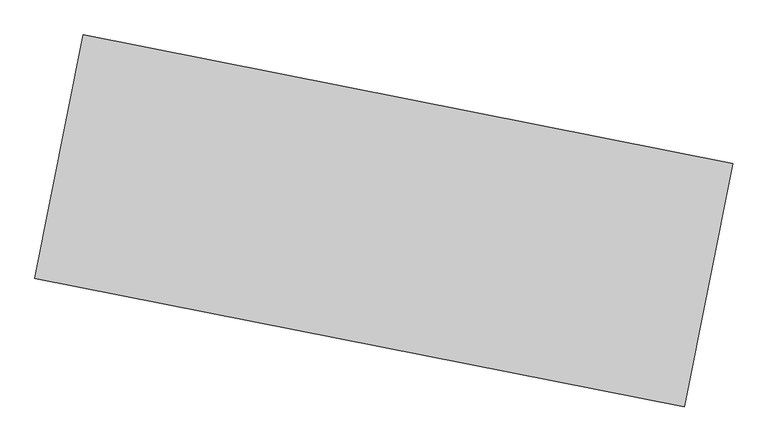
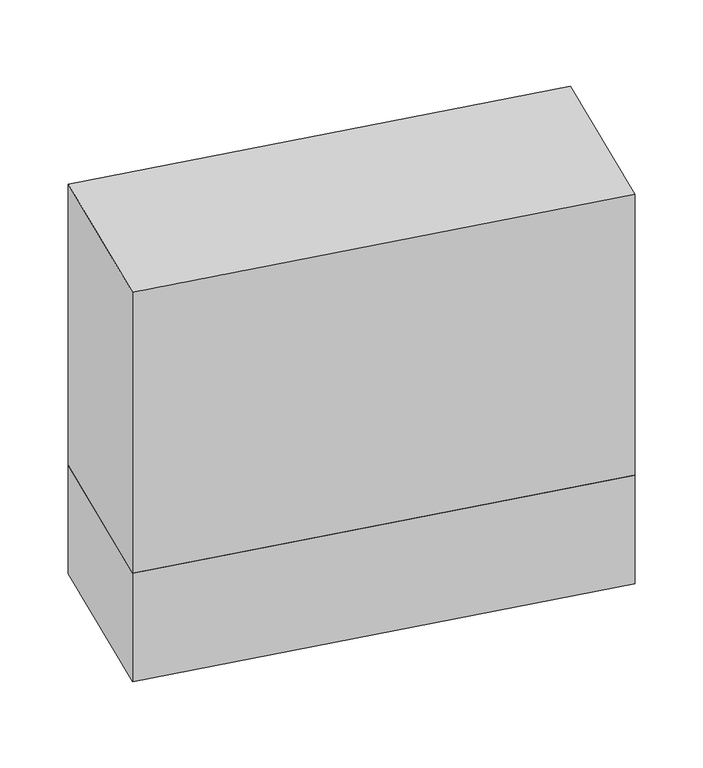
"""IFC4 building model written with IfcOpenShell, lengths in millimetres: furniture geometry, Monument sign2 : Monument sign."""

from ifc_helpers import new_model, si_unit, frame, origin, origin_with_axes, place, context, project, spatial, polyline, outline, extrude, source, transform, mapped, element, save


def furniture_524f5cd6(model_context):
    return source(origin(), model_context, "Body", "SweptSolid", [
        extrude(outline(polyline([(-3303.1352684, 235123.304702), (-911.1604416, 234649.7532396), (-1088.74224, 233752.7626795), (-3480.7170669, 234226.314142), (-3303.1352684, 235123.304702)])), origin_with_axes(), (0.0, 0.0, 1.0), 1574.8),
        extrude(outline(polyline([(-911.1604416, 234649.7532396), (-1088.74224, 233752.7626795), (-3480.7170669, 234226.314142), (-3303.1352684, 235123.304702), (-911.1604416, 234649.7532396)])), frame((0.0, 0.0, -609.6), z_axis=(0.0, 0.0, 1.0), x_axis=(1.0, 0.0, 0.0)), (0.0, 0.0, 1.0), 609.6),
    ])


if __name__ == "__main__":
    model = new_model("IFC4")
    model_context = context("Model", 3, world=origin())
    ifc_project = project(units=[si_unit("LENGTHUNIT", "METRE", prefix="MILLI")], contexts=[model_context])
    site = spatial("IfcSite", under=ifc_project)
    building = spatial("IfcBuilding", under=site)
    placement = place(None, origin())
    furniture_shape = furniture_524f5cd6(model_context)
    element("IfcFurniture", 1, ObjectType="Monument sign2 : Monument sign", at=placement, inside=building, context=model_context, shape_type="MappedRepresentation", body=[
        mapped(furniture_shape, transform((0.0, 0.0, 0.0), x_axis=(1.0, 0.0, 0.0), y_axis=(0.0, 1.0, 0.0), z_axis=(0.0, 0.0, 1.0))),
    ])
    save(model, "model.ifc")

# Revit data of these elements
# Element 1 (IfcFurniture, "Monument sign2 : Monument sign")
#   Materials on its faces: "COMPOSITE SIDING (WOOD GRAIN) - TO MATCH MAIN BUILDING", "METAL PANEL (DARK BRONZE) - TO MATCH MAIN BUILDING ACCENT METAL"
# Materials
#   "COMPOSITE SIDING (WOOD GRAIN) - TO MATCH MAIN BUILDING": class "Miscellaneous", colour RGB 143 84 44, transparency 0, Cost = 0
#   "METAL PANEL (DARK BRONZE) - TO MATCH MAIN BUILDING ACCENT METAL": class "Generic", colour RGB 88 62 61, transparency 0, Cost = 0
